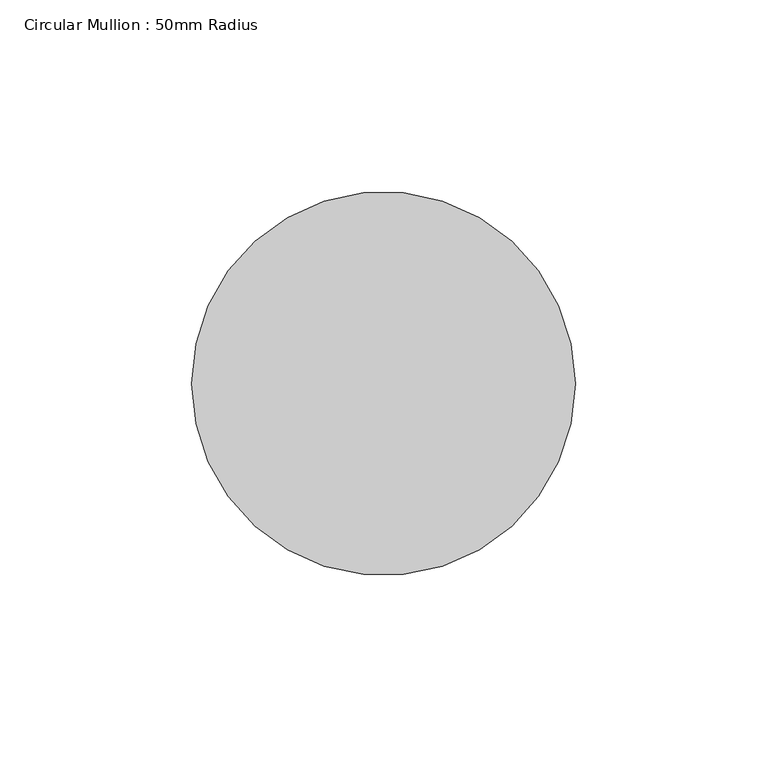
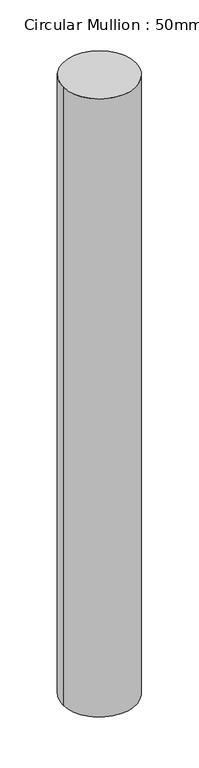
"""IFC4 building model written with IfcOpenShell, lengths in millimetres: member geometry, Circular Mullion : 50mm Radius."""

from ifc_helpers import new_model, si_unit, point, frame, origin, origin_2d, place, context, project, spatial, circle_curve, trimmed, segment, composite_curve, outline, extrude, source, transform, mapped, element, save


def circular_mullion_50mm_radius_c7c6d7dc(model_context):
    return source(origin(), model_context, "Body", "SweptSolid", [
        extrude(outline(composite_curve([segment(trimmed(circle_curve(origin_2d(), 50.0), [point((50.0, 0.0))], [point((-50.0, 0.0))], False, "CARTESIAN"), True, "CONTINUOUS"), segment(trimmed(circle_curve(origin_2d(), 50.0), [point((-50.0, 0.0))], [point((50.0, 0.0))], False, "CARTESIAN"), True, "CONTINUOUS")], self_intersect=False)), frame((0.0, 0.0, -898.3124149), z_axis=(0.0, 0.0, 1.0), x_axis=(1.0, 0.0, 0.0)), (0.0, 0.0, 1.0), 898.3124149),
    ])


if __name__ == "__main__":
    model = new_model("IFC4")
    model_context = context("Model", 3, world=origin())
    ifc_project = project(units=[si_unit("LENGTHUNIT", "METRE", prefix="MILLI")], contexts=[model_context])
    site = spatial("IfcSite", under=ifc_project)
    building = spatial("IfcBuilding", under=site)
    placement = place(None, origin())
    circular_mullion_50mm_radius_shape = circular_mullion_50mm_radius_c7c6d7dc(model_context)
    element("IfcMember", 1, ObjectType="Circular Mullion : 50mm Radius", at=placement, inside=building, context=model_context, shape_type="MappedRepresentation", body=[
        mapped(circular_mullion_50mm_radius_shape, transform((0.0, 0.0, 0.0), x_axis=(1.0, 0.0, 0.0), y_axis=(0.0, 1.0, 0.0), z_axis=(0.0, 0.0, 1.0))),
    ])
    save(model, "model.ifc")

# Revit data of these elements
# Type "Circular Mullion : 50mm Radius"
#   built-in parameter 1007350 = 0.164042 (stored number, unit not read)
# Element 1 (IfcMember, "Circular Mullion : 50mm Radius")
#   Materials on its faces: "Aluminium"
# Materials
#   "Aluminium": class "Metal", colour RGB 247 247 247, transparency 0, Description = "Aluminium 6061", Cost = 0
